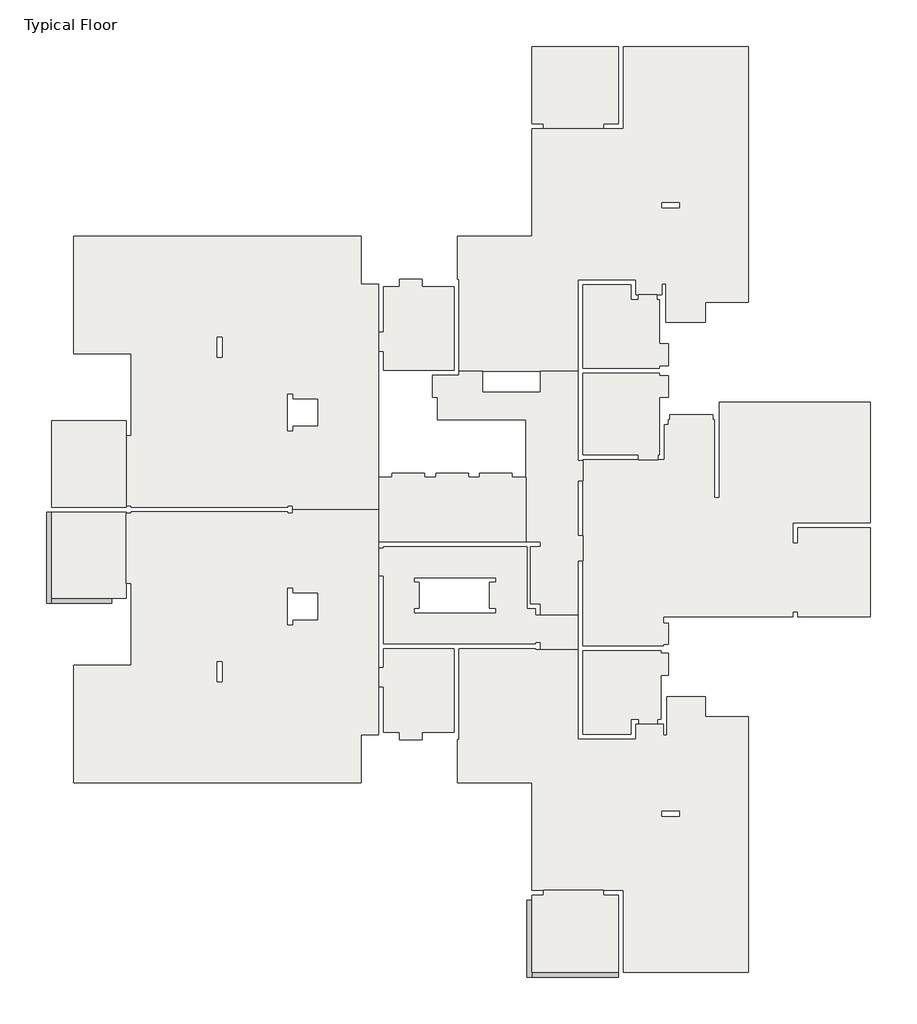
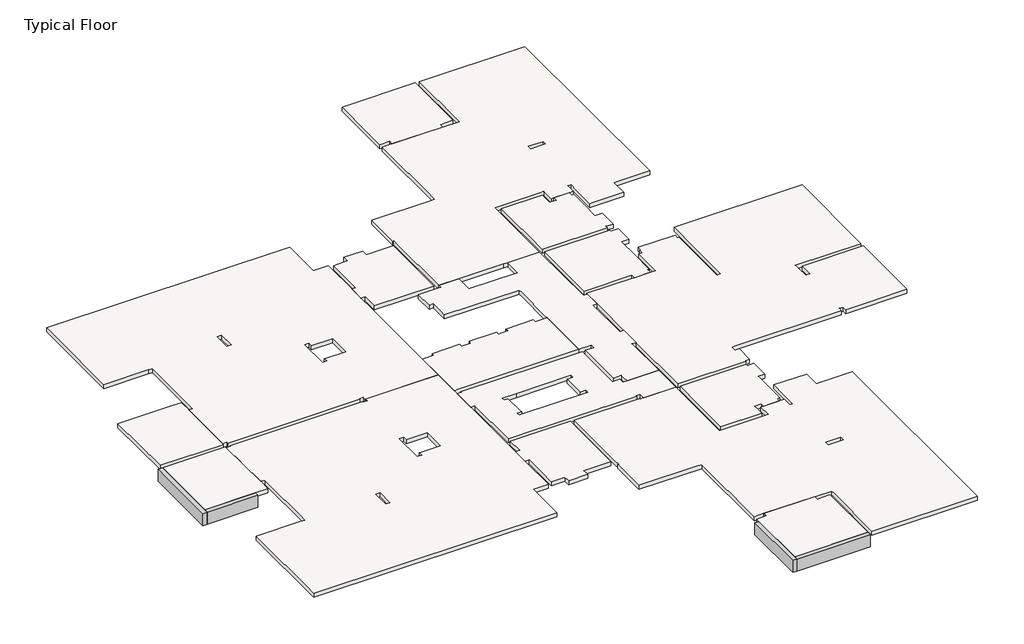
# One storey: 17 slabs, 4 beams.
"""IFC4 building model written with IfcOpenShell, lengths in millimetres."""

from ifc_helpers import new_model, si_unit, frame, origin, place, context, project, spatial, polyline, outline, extrude, faceted_brep, element, save

model = new_model("IFC4")

# Units and contexts
model_context = context("Model", 3, world=origin())
ifc_project = project(units=[si_unit("LENGTHUNIT", "METRE", prefix="MILLI")], contexts=[model_context])

# Site, building, storey
site = spatial("IfcSite", under=ifc_project)
building = spatial("IfcBuilding", under=site)
storey = spatial("IfcBuildingStorey", under=building, Name="Typical Floor", Elevation=3000.0)

# Beams
placement = place(None, origin())
element("IfcBeam", 1, ObjectType="Concrete Rectengular Beam : 20/60", at=placement, inside=storey, context=model_context, shape_type="Brep", body=[
    faceted_brep([(-15942.9172386, -82.3626254, 3000.0), (-15742.9172386, -82.3626254, 3000.0), (-15742.9172386, 117.6373746, 3000.0), (-15742.9172386, 3570.6507339, 3000.0), (-15942.9172386, 3570.6507339, 3000.0), (-15742.9172386, -82.3626254, 2400.0), (-15742.9172386, 117.6373746, 2400.0), (-15742.9172386, 3570.6507339, 2400.0), (-15742.9172386, 3570.6507339, 2800.0), (-15942.9172386, -82.3626254, 2400.0), (-15942.9172386, 3570.6507339, 2400.0)], [[[0, 1, 2, 3, 4]], [[1, 5, 6, 7, 8, 3, 2]], [[5, 9, 10, 7, 6]], [[9, 0, 4, 10]], [[1, 0, 9, 5]], [[4, 3, 8, 7, 10]]]),
])
element("IfcBeam", 2, ObjectType="Concrete Rectengular Beam : 20/60", at=placement, inside=storey, context=model_context, shape_type="Brep", body=[
    faceted_brep([(-15742.9172386, 117.6373746, 3000.0), (-15742.9172386, -82.3626254, 3000.0), (-13340.0412254, -82.3626254, 3000.0), (-13340.0412254, 117.6373746, 3000.0), (-15742.9172386, 117.6373746, 2400.0), (-15742.9172386, 117.6373746, 2800.0), (-13340.0412254, 117.6373746, 2400.0), (-15742.9172386, -82.3626254, 2400.0), (-13340.0412254, -82.3626254, 2400.0)], [[[0, 1, 2, 3]], [[4, 5, 0, 3, 6]], [[7, 4, 6, 8]], [[8, 2, 1, 7]], [[1, 0, 5, 4, 7]], [[3, 2, 8, 6]]]),
])
element("IfcBeam", 3, ObjectType="Concrete Rectengular Beam : 20/60", at=placement, inside=storey, context=model_context, shape_type="Brep", body=[
    faceted_brep([(3325.3580541, -15077.7243787, 3000.0), (3525.3580541, -15077.7243787, 3000.0), (3525.3580541, -14877.7243787, 3000.0), (3525.3580541, -11977.8894943, 3000.0), (3325.3580541, -11977.8894943, 3000.0), (3525.3580541, -15077.7243787, 2400.0), (3525.3580541, -14877.7243787, 2400.0), (3525.3580541, -11977.8894943, 2400.0), (3325.3580541, -15077.7243787, 2400.0), (3325.3580541, -11977.8894943, 2400.0)], [[[0, 1, 2, 3, 4]], [[1, 5, 6, 7, 3, 2]], [[5, 8, 9, 7, 6]], [[8, 0, 4, 9]], [[1, 0, 8, 5]], [[4, 3, 7, 9]]]),
])
element("IfcBeam", 4, ObjectType="Concrete Rectengular Beam : 20/60", at=placement, inside=storey, context=model_context, shape_type="Brep", body=[
    faceted_brep([(6985.0248209, -15077.7243787, 3000.0), (6985.0248209, -14877.7243787, 3000.0), (3525.3580541, -14877.7243787, 3000.0), (3525.3580541, -15077.7243787, 3000.0), (6985.0248209, -14877.7243787, 2800.0), (6985.0248209, -14877.7243787, 2400.0), (3525.3580541, -14877.7243787, 2400.0), (3525.3580541, -14877.7243787, 2800.0), (6985.0248209, -15077.7243787, 2400.0), (3525.3580541, -15077.7243787, 2400.0)], [[[0, 1, 2, 3]], [[1, 4, 5, 6, 7, 2]], [[5, 8, 9, 6]], [[8, 0, 3, 9]], [[1, 0, 8, 5, 4]], [[3, 2, 7, 6, 9]]]),
])

# Slabs
element("IfcSlab", 5, ObjectType="20", at=placement, inside=storey, context=model_context, shape_type="Brep", body=[
    faceted_brep([(-12744.8761098, 117.6373746, 2800.0), (-15742.9172386, 117.6373746, 2800.0), (-15742.9172386, 3570.6507339, 2800.0), (-12745.0412254, 3570.6507339, 2800.0), (-12745.0412254, 3522.8272575, 2800.0), (-12744.8761098, 3522.8272575, 2800.0), (-12744.8761098, 723.063673, 2800.0), (-15742.9172386, 117.6373746, 3000.0), (-13340.0412254, 117.6373746, 3000.0), (-12744.8761098, 117.6373746, 3000.0), (-12744.8761098, 723.063673, 3000.0), (-12744.8761098, 3522.8272575, 3000.0), (-12745.0412254, 3522.8272575, 3000.0), (-12745.0412254, 3570.6507339, 3000.0), (-15742.9172386, 3570.6507339, 3000.0)], [[[0, 1, 2, 3, 4, 5, 6]], [[7, 8, 9, 10, 11, 12, 13, 14]], [[9, 0, 6, 5, 11, 10]], [[1, 0, 9, 8, 7]], [[2, 1, 7, 14]], [[2, 14, 13, 3]], [[12, 4, 3, 13]], [[4, 12, 11, 5]]]),
])
element("IfcSlab", 6, ObjectType="20", at=placement, inside=storey, context=model_context, shape_type="Brep", body=[
    faceted_brep([(-15742.9172386, 3770.6507339, 2800.0), (-15742.9172386, 7228.4299293, 2800.0), (-12744.8761098, 7228.4299293, 2800.0), (-12744.8761098, 6623.0036309, 2800.0), (-12742.9172386, 6623.0036309, 2800.0), (-12742.9172386, 3823.2400464, 2800.0), (-12742.9172386, 3818.3090948, 2800.0), (-12745.0412254, 3818.3090948, 2800.0), (-12745.0412254, 3770.6507339, 2800.0), (-15742.9172386, 7228.4299293, 3000.0), (-15742.9172386, 3770.6507339, 3000.0), (-12745.0412254, 3770.6507339, 3000.0), (-12745.0412254, 3818.3090948, 3000.0), (-12742.9172386, 3818.3090948, 3000.0), (-12742.9172386, 3823.2400464, 3000.0), (-12742.9172386, 6623.0036309, 3000.0), (-12744.8761098, 6623.0036309, 3000.0), (-12744.8761098, 7228.4299293, 3000.0), (-13340.0412254, 7228.4299293, 3000.0)], [[[0, 1, 2, 3, 4, 5, 6, 7, 8]], [[9, 10, 11, 12, 13, 14, 15, 16, 17, 18]], [[4, 15, 14, 13, 6, 5]], [[10, 0, 8, 11]], [[1, 0, 10, 9]], [[1, 9, 18, 17, 2]], [[16, 3, 2, 17]], [[3, 16, 15, 4]], [[7, 12, 11, 8]], [[12, 7, 6, 13]]]),
])
element("IfcSlab", 7, ObjectType="20", at=placement, inside=storey, context=model_context, shape_type="Brep", body=[
    faceted_brep([(-12744.8761098, 3522.8272575, 2800.0), (-12545.0412254, 3522.8272575, 2800.0), (-12545.0412254, 3573.033652, 2800.0), (-6284.9504118, 3573.033652, 2800.0), (-6284.9504118, 3522.8272575, 2800.0), (-6084.9504118, 3522.8272575, 2800.0), (-6084.9504118, 3672.9510942, 2800.0), (-2634.3199705, 3672.9510942, 2800.0), (-2634.3199705, 2374.2607609, 2800.0), (-2634.3199705, 2124.0543665, 2800.0), (-2634.3199705, 1012.4872695, 2800.0), (-2634.3199705, -2660.6799476, 2800.0), (-2634.3199705, -3430.3624753, 2800.0), (-2634.3199705, -5346.2285816, 2800.0), (-3134.897875, -5346.2285816, 2800.0), (-3334.897875, -5346.2285816, 2800.0), (-3334.897875, -7276.5573117, 2800.0), (-14851.7058906, -7276.5573117, 2800.0), (-14851.7058906, -2576.5573117, 2800.0), (-12744.8761098, -2576.5573117, 2800.0), (-12744.8761098, -2576.936327, 2800.0), (-12544.8761098, -2576.936327, 2800.0), (-12544.8761098, 723.063673, 2800.0), (-12744.8761098, 723.063673, 2800.0), (-8908.7851697, -2433.7684532, 2800.0), (-9108.7851697, -2433.7684532, 2800.0), (-9108.7851697, -3233.7684532, 2800.0), (-8908.7851697, -3233.7684532, 2800.0), (-6084.7852962, 522.8985574, 2800.0), (-6284.7852962, 522.8985574, 2800.0), (-6284.7852962, -947.1014426, 2800.0), (-6084.7852962, -947.1014426, 2800.0), (-6084.7852962, -744.8138413, 2800.0), (-5083.9597183, -744.8138413, 2800.0), (-5083.9597183, 322.7334418, 2800.0), (-6084.7852962, 322.7334418, 2800.0), (-12545.0412254, 3522.8272575, 3000.0), (-12744.8761098, 3522.8272575, 3000.0), (-12744.8761098, 723.063673, 3000.0), (-12544.8761098, 723.063673, 3000.0), (-12544.8761098, -2576.936327, 3000.0), (-12744.8761098, -2576.936327, 3000.0), (-12744.8761098, -2576.5573117, 3000.0), (-14851.7058906, -2576.5573117, 3000.0), (-14851.7058906, -7276.5573117, 3000.0), (-3334.897875, -7276.5573117, 3000.0), (-3334.897875, -5346.2285816, 3000.0), (-3134.897875, -5346.2285816, 3000.0), (-2634.3199705, -5346.2285816, 3000.0), (-2634.3199705, -3430.3624753, 3000.0), (-2634.3199705, -2660.6799476, 3000.0), (-2634.3199705, 1012.4872695, 3000.0), (-2634.3199705, 2124.0543665, 3000.0), (-2634.3199705, 2374.2607609, 3000.0), (-2634.3199705, 3672.9510942, 3000.0), (-6084.9504118, 3672.9510942, 3000.0), (-6084.9504118, 3522.8272575, 3000.0), (-6284.9504118, 3522.8272575, 3000.0), (-6284.9504118, 3573.033652, 3000.0), (-12545.0412254, 3573.033652, 3000.0), (-9108.7851697, -2433.7684532, 3000.0), (-8908.7851697, -2433.7684532, 3000.0), (-8908.7851697, -3233.7684532, 3000.0), (-9108.7851697, -3233.7684532, 3000.0), (-6284.7852962, 522.8985574, 3000.0), (-6084.7852962, 522.8985574, 3000.0), (-6084.7852962, 322.7334418, 3000.0), (-5083.9597183, 322.7334418, 3000.0), (-5083.9597183, -744.8138413, 3000.0), (-6084.7852962, -744.8138413, 3000.0), (-6084.7852962, -947.1014426, 3000.0), (-6284.7852962, -947.1014426, 3000.0)], [[[0, 1, 2, 3, 4, 5, 6, 7, 8, 9, 10, 11, 12, 13, 14, 15, 16, 17, 18, 19, 20, 21, 22, 23], [24, 25, 26, 27], [28, 29, 30, 31, 32, 33, 34, 35]], [[36, 37, 38, 39, 40, 41, 42, 43, 44, 45, 46, 47, 48, 49, 50, 51, 52, 53, 54, 55, 56, 57, 58, 59], [60, 61, 62, 63], [64, 65, 66, 67, 68, 69, 70, 71]], [[1, 0, 37, 36]], [[2, 1, 36, 59]], [[3, 2, 59, 58]], [[4, 3, 58, 57]], [[5, 4, 57, 56]], [[6, 5, 56, 55]], [[7, 6, 55, 54]], [[13, 12, 11, 10, 9, 8, 7, 54, 53, 52, 51, 50, 49, 48]], [[13, 48, 47, 46, 15, 14]], [[15, 46, 45, 16]], [[43, 18, 17, 44]], [[18, 43, 42, 19]], [[38, 23, 22, 39]], [[0, 23, 38, 37]], [[25, 24, 61, 60]], [[26, 25, 60, 63]], [[27, 26, 63, 62]], [[24, 27, 62, 61]], [[29, 28, 65, 64]], [[30, 29, 64, 71]], [[31, 30, 71, 70]], [[32, 31, 70, 69]], [[33, 32, 69, 68]], [[34, 33, 68, 67]], [[35, 34, 67, 66]], [[28, 35, 66, 65]], [[21, 40, 39, 22]], [[41, 20, 19, 42]], [[40, 21, 20, 41]], [[17, 16, 45, 44]]]),
])
element("IfcSlab", 8, ObjectType="20", at=placement, inside=storey, context=model_context, shape_type="Brep", body=[
    faceted_brep([(-6284.9504118, 3773.033652, 2800.0), (-12545.0412254, 3773.033652, 2800.0), (-12545.0412254, 3818.3090948, 2800.0), (-12545.0412254, 3823.2400464, 2800.0), (-12742.9172386, 3823.2400464, 2800.0), (-12742.9172386, 6623.0036309, 2800.0), (-12544.8761098, 6623.0036309, 2800.0), (-12544.8761098, 9923.0036309, 2800.0), (-12744.8761098, 9923.0036309, 2800.0), (-12744.8761098, 9922.6246156, 2800.0), (-14851.7058906, 9922.6246156, 2800.0), (-14851.7058906, 14622.6246156, 2800.0), (-3334.897875, 14622.6246156, 2800.0), (-3334.897875, 12692.2958855, 2800.0), (-3134.897875, 12692.2958855, 2800.0), (-2634.3199705, 12692.2958855, 2800.0), (-2634.3199705, 10776.4297792, 2800.0), (-2634.3199705, 10006.7472515, 2800.0), (-2634.3199705, 4974.0243454, 2800.0), (-2634.3199705, 3672.9510942, 2800.0), (-6084.9504118, 3672.9510942, 2800.0), (-6084.9504118, 3823.2400464, 2800.0), (-6284.9504118, 3823.2400464, 2800.0), (-9108.7851697, 9779.8357571, 2800.0), (-8908.7851697, 9779.8357571, 2800.0), (-8908.7851697, 10579.8357571, 2800.0), (-9108.7851697, 10579.8357571, 2800.0), (-6284.7852962, 6823.1687465, 2800.0), (-6084.7852962, 6823.1687465, 2800.0), (-6084.7852962, 7023.3338621, 2800.0), (-5083.9597183, 7023.3338621, 2800.0), (-5083.9597183, 8090.8811452, 2800.0), (-6084.7852962, 8090.8811452, 2800.0), (-6084.7852962, 8293.1687465, 2800.0), (-6284.7852962, 8293.1687465, 2800.0), (-12545.0412254, 3773.033652, 3000.0), (-6284.9504118, 3773.033652, 3000.0), (-6284.9504118, 3823.2400464, 3000.0), (-6084.9504118, 3823.2400464, 3000.0), (-6084.9504118, 3672.9510942, 3000.0), (-2634.3199705, 3672.9510942, 3000.0), (-2634.3199705, 4974.0243454, 3000.0), (-2634.3199705, 5124.0243454, 3000.0), (-2634.3199705, 7974.2832767, 3000.0), (-2634.3199705, 8174.2832767, 3000.0), (-2634.3199705, 9053.5800344, 3000.0), (-2634.3199705, 9253.5800344, 3000.0), (-2634.3199705, 10006.7472515, 3000.0), (-2634.3199705, 10776.4297792, 3000.0), (-2634.3199705, 12692.2958855, 3000.0), (-3134.897875, 12692.2958855, 3000.0), (-3334.897875, 12692.2958855, 3000.0), (-3334.897875, 14622.6246156, 3000.0), (-14851.7058906, 14622.6246156, 3000.0), (-14851.7058906, 9922.6246156, 3000.0), (-12744.8761098, 9922.6246156, 3000.0), (-12744.8761098, 9923.0036309, 3000.0), (-12544.8761098, 9923.0036309, 3000.0), (-12544.8761098, 6623.0036309, 3000.0), (-12742.9172386, 6623.0036309, 3000.0), (-12742.9172386, 3823.2400464, 3000.0), (-12545.0412254, 3823.2400464, 3000.0), (-12545.0412254, 3818.3090948, 3000.0), (-8908.7851697, 9779.8357571, 3000.0), (-9108.7851697, 9779.8357571, 3000.0), (-9108.7851697, 10579.8357571, 3000.0), (-8908.7851697, 10579.8357571, 3000.0), (-6084.7852962, 6823.1687465, 3000.0), (-6284.7852962, 6823.1687465, 3000.0), (-6284.7852962, 8293.1687465, 3000.0), (-6084.7852962, 8293.1687465, 3000.0), (-6084.7852962, 8090.8811452, 3000.0), (-5083.9597183, 8090.8811452, 3000.0), (-5083.9597183, 7023.3338621, 3000.0), (-6084.7852962, 7023.3338621, 3000.0)], [[[0, 1, 2, 3, 4, 5, 6, 7, 8, 9, 10, 11, 12, 13, 14, 15, 16, 17, 18, 19, 20, 21, 22], [23, 24, 25, 26], [27, 28, 29, 30, 31, 32, 33, 34]], [[35, 36, 37, 38, 39, 40, 41, 42, 43, 44, 45, 46, 47, 48, 49, 50, 51, 52, 53, 54, 55, 56, 57, 58, 59, 60, 61, 62], [63, 64, 65, 66], [67, 68, 69, 70, 71, 72, 73, 74]], [[3, 61, 60, 4]], [[1, 35, 62, 61, 3, 2]], [[1, 0, 36, 35]], [[0, 22, 37, 36]], [[22, 21, 38, 37]], [[21, 20, 39, 38]], [[20, 19, 40, 39]], [[19, 18, 17, 16, 15, 49, 48, 47, 46, 45, 44, 43, 42, 41, 40]], [[13, 51, 50, 49, 15, 14]], [[51, 13, 12, 52]], [[10, 54, 53, 11]], [[54, 10, 9, 55]], [[58, 6, 5, 59]], [[24, 23, 64, 63]], [[23, 26, 65, 64]], [[26, 25, 66, 65]], [[25, 24, 63, 66]], [[28, 27, 68, 67]], [[27, 34, 69, 68]], [[34, 33, 70, 69]], [[33, 32, 71, 70]], [[32, 31, 72, 71]], [[31, 30, 73, 72]], [[30, 29, 74, 73]], [[29, 28, 67, 74]], [[8, 56, 55, 9]], [[6, 58, 57, 7]], [[7, 57, 56, 8]], [[5, 4, 60, 59]], [[12, 11, 53, 52]]]),
])
element("IfcSlab", 9, ObjectType="20", at=placement, inside=storey, context=model_context, shape_type="SweptSolid", body=[
    extrude(outline(polyline([(-2434.3199705, -2660.6799476), (-2434.3199705, -1909.5654174), (385.0023051, -1909.5654174), (385.0023051, -5246.2285816), (-885.2581272, -5246.2285816), (-885.2581272, -5546.2285816), (-1781.9370524, -5546.2285816), (-1781.9370524, -5246.2285816), (-2434.3199705, -5246.2285816), (-2434.3199705, -3430.3624753), (-2634.3199705, -3430.3624753), (-2634.3199705, -2660.6799476), (-2434.3199705, -2660.6799476)])), frame((0.0, 0.0, 2800.0), z_axis=(0.0, 0.0, 1.0), x_axis=(1.0, 0.0, 0.0)), (0.0, 0.0, 1.0), 200.0),
])
element("IfcSlab", 10, ObjectType="20", at=placement, inside=storey, context=model_context, shape_type="Brep", body=[
    faceted_brep([(3654.3658596, -1909.5654174, 2800.0), (3654.3658596, -1955.5013225, 2800.0), (3854.3658596, -1955.5013225, 2800.0), (5355.6042265, -1955.5013225, 2800.0), (5355.6042265, -5329.7132709, 2800.0), (5355.6042265, -5529.7132709, 2800.0), (7481.1671205, -5529.7132709, 2800.0), (7681.1671205, -5529.7132709, 2800.0), (7681.1671205, -4929.2179242, 2800.0), (7809.9023103, -4929.2179242, 2800.0), (8554.8987326, -4929.2179242, 2800.0), (8779.8987326, -4929.2179242, 2800.0), (8779.8987326, -5377.2065162, 2800.0), (8929.8987326, -5377.2065162, 2800.0), (8929.8987326, -4829.2179242, 2800.0), (8929.8987326, -3825.7617548, 2800.0), (10478.8780181, -3825.7617548, 2800.0), (10478.8780181, -4426.5873327, 2800.0), (10478.8780181, -4626.5873327, 2800.0), (12185.0248209, -4626.5873327, 2800.0), (12185.0248209, -14877.7243787, 2800.0), (7185.0248209, -14877.7243787, 2800.0), (7185.0248209, -11777.7243787, 2800.0), (7185.0248209, -11577.7243787, 2800.0), (6385.0248209, -11577.7243787, 2800.0), (3983.0434339, -11577.7243787, 2800.0), (3525.3580541, -11577.7243787, 2800.0), (3525.3580541, -7276.5573117, 2800.0), (539.5617467, -7276.5573117, 2800.0), (539.5617467, -5546.2285816, 2800.0), (585.0023051, -5546.2285816, 2800.0), (585.0023051, -5246.2285816, 2800.0), (585.0023051, -1909.5654174, 2800.0), (9430.3940793, -8427.3416107, 2800.0), (8730.3940793, -8427.3416107, 2800.0), (8730.3940793, -8627.3416107, 2800.0), (9430.3940793, -8627.3416107, 2800.0), (3654.3658596, -1955.5013225, 3000.0), (3654.3658596, -1909.5654174, 3000.0), (585.0023051, -1909.5654174, 3000.0), (585.0023051, -5246.2285816, 3000.0), (585.0023051, -5546.2285816, 3000.0), (539.5617467, -5546.2285816, 3000.0), (539.5617467, -7276.5573117, 3000.0), (3325.3580541, -7276.5573117, 3000.0), (3525.3580541, -7276.5573117, 3000.0), (3525.3580541, -11577.7243787, 3000.0), (3983.0434339, -11577.7243787, 3000.0), (6385.0248209, -11577.7243787, 3000.0), (7185.0248209, -11577.7243787, 3000.0), (7185.0248209, -11777.7243787, 3000.0), (7185.0248209, -14877.7243787, 3000.0), (12185.0248209, -14877.7243787, 3000.0), (12185.0248209, -4626.5873327, 3000.0), (10478.8780181, -4626.5873327, 3000.0), (10478.8780181, -4426.5873327, 3000.0), (10478.8780181, -3825.7617548, 3000.0), (8929.8987326, -3825.7617548, 3000.0), (8929.8987326, -4829.2179242, 3000.0), (8929.8987326, -5377.2065162, 3000.0), (8779.8987326, -5377.2065162, 3000.0), (8779.8987326, -4929.2179242, 3000.0), (8554.8987326, -4929.2179242, 3000.0), (7809.9023103, -4929.2179242, 3000.0), (7681.1671205, -4929.2179242, 3000.0), (7681.1671205, -5529.7132709, 3000.0), (7481.1671205, -5529.7132709, 3000.0), (5355.6042265, -5529.7132709, 3000.0), (5355.6042265, -5329.7132709, 3000.0), (5355.6042265, -1955.5013225, 3000.0), (3854.3658596, -1955.5013225, 3000.0), (8730.3940793, -8427.3416107, 3000.0), (9430.3940793, -8427.3416107, 3000.0), (9430.3940793, -8627.3416107, 3000.0), (8730.3940793, -8627.3416107, 3000.0)], [[[0, 1, 2, 3, 4, 5, 6, 7, 8, 9, 10, 11, 12, 13, 14, 15, 16, 17, 18, 19, 20, 21, 22, 23, 24, 25, 26, 27, 28, 29, 30, 31, 32], [33, 34, 35, 36]], [[37, 38, 39, 40, 41, 42, 43, 44, 45, 46, 47, 48, 49, 50, 51, 52, 53, 54, 55, 56, 57, 58, 59, 60, 61, 62, 63, 64, 65, 66, 67, 68, 69, 70], [71, 72, 73, 74]], [[1, 0, 38, 37]], [[2, 1, 37, 70]], [[3, 2, 70, 69]], [[3, 69, 68, 67, 5, 4]], [[5, 67, 66, 65, 7, 6]], [[8, 7, 65, 64]], [[8, 64, 63, 62, 61, 11, 10, 9]], [[12, 11, 61, 60]], [[13, 12, 60, 59]], [[13, 59, 58, 57, 15, 14]], [[16, 15, 57, 56]], [[16, 56, 55, 54, 18, 17]], [[19, 18, 54, 53]], [[20, 19, 53, 52]], [[21, 20, 52, 51]], [[21, 51, 50, 49, 23, 22]], [[24, 23, 49, 48]], [[25, 24, 48, 47]], [[26, 25, 47, 46]], [[26, 46, 45, 27]], [[42, 29, 28, 43]], [[30, 29, 42, 41]], [[30, 41, 40, 39, 32, 31]], [[0, 32, 39, 38]], [[34, 33, 72, 71]], [[35, 34, 71, 74]], [[36, 35, 74, 73]], [[33, 36, 73, 72]], [[27, 45, 44, 43, 28]]]),
])
element("IfcSlab", 11, ObjectType="20", at=placement, inside=storey, context=model_context, shape_type="Brep", body=[
    faceted_brep([(3983.0434339, -11777.7243787, 2800.0), (3983.0434339, -11577.7243787, 2800.0), (6385.0248209, -11577.7243787, 2800.0), (6385.0248209, -11777.7243787, 2800.0), (6985.0248209, -11777.7243787, 2800.0), (6985.0248209, -14877.7243787, 2800.0), (3525.3580541, -14877.7243787, 2800.0), (3525.3580541, -11777.7243787, 2800.0), (3983.0434339, -11577.7243787, 3000.0), (3983.0434339, -11777.7243787, 3000.0), (3525.3580541, -11777.7243787, 3000.0), (3525.3580541, -11977.8894943, 3000.0), (3525.3580541, -14877.7243787, 3000.0), (6985.0248209, -14877.7243787, 3000.0), (6985.0248209, -11777.7243787, 3000.0), (6385.0248209, -11777.7243787, 3000.0), (6385.0248209, -11577.7243787, 3000.0)], [[[0, 1, 2, 3, 4, 5, 6, 7]], [[8, 9, 10, 11, 12, 13, 14, 15, 16]], [[1, 0, 9, 8]], [[2, 1, 8, 16]], [[3, 2, 16, 15]], [[4, 3, 15, 14]], [[5, 4, 14, 13]], [[6, 5, 13, 12]], [[7, 6, 12, 11, 10]], [[0, 7, 10, 9]]]),
])
element("IfcSlab", 12, ObjectType="20", at=placement, inside=storey, context=model_context, shape_type="Brep", body=[
    faceted_brep([(8680.0225693, -4729.2179242, 2800.0), (8554.8987326, -4729.2179242, 2800.0), (8554.8987326, -4929.2179242, 2800.0), (7809.9023103, -4929.2179242, 2800.0), (7809.9023103, -4729.2179242, 2800.0), (7481.1671205, -4729.2179242, 2800.0), (7481.1671205, -4929.2179242, 2800.0), (7481.1671205, -5329.7132709, 2800.0), (5555.6042265, -5329.7132709, 2800.0), (5555.6042265, -1979.0002718, 2800.0), (8679.7748959, -1979.0002718, 2800.0), (8679.7748959, -2077.0301427, 2800.0), (8979.7748959, -2077.0301427, 2800.0), (8979.7748959, -2977.6080472, 2800.0), (8679.7748959, -2977.6080472, 2800.0), (8679.7748959, -3625.7617548, 2800.0), (8680.0225693, -3625.7617548, 2800.0), (8680.0225693, -3825.7617548, 2800.0), (8554.8987326, -4729.2179242, 3000.0), (8680.0225693, -4729.2179242, 3000.0), (8680.0225693, -3825.7617548, 3000.0), (8680.0225693, -3625.7617548, 3000.0), (8679.7748959, -3625.7617548, 3000.0), (8679.7748959, -2977.6080472, 3000.0), (8979.7748959, -2977.6080472, 3000.0), (8979.7748959, -2077.0301427, 3000.0), (8679.7748959, -2077.0301427, 3000.0), (8679.7748959, -1979.0002718, 3000.0), (5555.6042265, -1979.0002718, 3000.0), (5555.6042265, -5329.7132709, 3000.0), (7481.1671205, -5329.7132709, 3000.0), (7481.1671205, -4929.2179242, 3000.0), (7481.1671205, -4729.2179242, 3000.0), (7809.9023103, -4729.2179242, 3000.0), (7809.9023103, -4929.2179242, 3000.0), (8554.8987326, -4929.2179242, 3000.0)], [[[0, 1, 2, 3, 4, 5, 6, 7, 8, 9, 10, 11, 12, 13, 14, 15, 16, 17]], [[18, 19, 20, 21, 22, 23, 24, 25, 26, 27, 28, 29, 30, 31, 32, 33, 34, 35]], [[19, 0, 17, 16, 21, 20]], [[1, 0, 19, 18]], [[2, 1, 18, 35]], [[3, 2, 35, 34]], [[4, 3, 34, 33]], [[5, 4, 33, 32]], [[5, 32, 31, 30, 7, 6]], [[8, 7, 30, 29]], [[9, 8, 29, 28]], [[10, 9, 28, 27]], [[11, 10, 27, 26]], [[12, 11, 26, 25]], [[13, 12, 25, 24]], [[13, 24, 23, 14]], [[14, 23, 22, 15]], [[15, 22, 21, 16]]]),
])
element("IfcSlab", 13, ObjectType="20", at=placement, inside=storey, context=model_context, shape_type="SweptSolid", body=[
    extrude(outline(polyline([(-885.2581272, 12592.2958855), (385.0023051, 12592.2958855), (385.0023051, 9253.5800344), (-2434.3199705, 9253.5800344), (-2434.3199705, 10006.7472515), (-2634.3199705, 10006.7472515), (-2634.3199705, 10776.4297792), (-2434.3199705, 10776.4297792), (-2434.3199705, 12592.2958855), (-1781.9370524, 12592.2958855), (-1781.9370524, 12892.2958855), (-885.2581272, 12892.2958855), (-885.2581272, 12592.2958855)])), frame((0.0, 0.0, 2800.0), z_axis=(0.0, 0.0, 1.0), x_axis=(1.0, 0.0, 0.0)), (0.0, 0.0, 1.0), 200.0),
])
element("IfcSlab", 14, ObjectType="20", at=placement, inside=storey, context=model_context, shape_type="Brep", body=[
    faceted_brep([(3854.3658596, 9203.7038711, 2800.0), (3654.3658596, 9203.7038711, 2800.0), (1535.7866041, 9203.7038711, 2800.0), (585.0023051, 9203.7038711, 2800.0), (585.0023051, 12592.2958855, 2800.0), (585.0023051, 12892.2958855, 2800.0), (539.5617467, 12892.2958855, 2800.0), (539.5617467, 14622.6246156, 2800.0), (3525.3580541, 14622.6246156, 2800.0), (3525.3580541, 18923.7916826, 2800.0), (3983.0434339, 18923.7916826, 2800.0), (6385.0248209, 18923.7916826, 2800.0), (7185.0248209, 18923.7916826, 2800.0), (7185.0248209, 19123.7916826, 2800.0), (7185.0248209, 22223.7916826, 2800.0), (12185.0248209, 22223.7916826, 2800.0), (12185.0248209, 11972.6546366, 2800.0), (10478.8780181, 11972.6546366, 2800.0), (10478.8780181, 11772.6546366, 2800.0), (10478.8780181, 11171.8290587, 2800.0), (8979.733617, 11171.8290587, 2800.0), (8879.6510592, 11171.8290587, 2800.0), (8879.6510592, 12075.1201125, 2800.0), (8879.6510592, 12275.1201125, 2800.0), (8879.6510592, 12723.2738201, 2800.0), (8729.6510592, 12723.2738201, 2800.0), (8729.6510592, 12275.1201125, 2800.0), (8530.0225693, 12275.1201125, 2800.0), (8530.0225693, 12270.1201125, 2800.0), (7795.7123021, 12270.1201125, 2800.0), (7795.7123021, 12275.2852281, 2800.0), (7681.1671205, 12275.2852281, 2800.0), (7681.1671205, 12875.7805748, 2800.0), (7481.1671205, 12875.7805748, 2800.0), (5355.6042265, 12875.7805748, 2800.0), (5355.6042265, 12675.7805748, 2800.0), (5355.6042265, 9203.7038711, 2800.0), (8730.3940793, 15773.4089146, 2800.0), (9430.3940793, 15773.4089146, 2800.0), (9430.3940793, 15973.4089146, 2800.0), (8730.3940793, 15973.4089146, 2800.0), (3654.3658596, 9203.7038711, 3000.0), (3854.3658596, 9203.7038711, 3000.0), (5355.6042265, 9203.7038711, 3000.0), (5355.6042265, 12675.7805748, 3000.0), (5355.6042265, 12875.7805748, 3000.0), (7481.1671205, 12875.7805748, 3000.0), (7681.1671205, 12875.7805748, 3000.0), (7681.1671205, 12275.2852281, 3000.0), (7795.7123021, 12275.2852281, 3000.0), (7795.7123021, 12270.1201125, 3000.0), (8530.0225693, 12270.1201125, 3000.0), (8530.0225693, 12275.1201125, 3000.0), (8729.6510592, 12275.1201125, 3000.0), (8729.6510592, 12723.2738201, 3000.0), (8879.6510592, 12723.2738201, 3000.0), (8879.6510592, 12275.1201125, 3000.0), (8879.6510592, 12075.1201125, 3000.0), (8879.6510592, 11171.8290587, 3000.0), (8979.733617, 11171.8290587, 3000.0), (10478.8780181, 11171.8290587, 3000.0), (10478.8780181, 11772.6546366, 3000.0), (10478.8780181, 11972.6546366, 3000.0), (12185.0248209, 11972.6546366, 3000.0), (12185.0248209, 22223.7916826, 3000.0), (7185.0248209, 22223.7916826, 3000.0), (7185.0248209, 19123.7916826, 3000.0), (7185.0248209, 18923.7916826, 3000.0), (6385.0248209, 18923.7916826, 3000.0), (3983.0434339, 18923.7916826, 3000.0), (3525.3580541, 18923.7916826, 3000.0), (3525.3580541, 14622.6246156, 3000.0), (3325.3580541, 14622.6246156, 3000.0), (539.5617467, 14622.6246156, 3000.0), (539.5617467, 12892.2958855, 3000.0), (585.0023051, 12892.2958855, 3000.0), (585.0023051, 12592.2958855, 3000.0), (585.0023051, 9203.7038711, 3000.0), (1535.7866041, 9203.7038711, 3000.0), (9430.3940793, 15773.4089146, 3000.0), (8730.3940793, 15773.4089146, 3000.0), (8730.3940793, 15973.4089146, 3000.0), (9430.3940793, 15973.4089146, 3000.0)], [[[0, 1, 2, 3, 4, 5, 6, 7, 8, 9, 10, 11, 12, 13, 14, 15, 16, 17, 18, 19, 20, 21, 22, 23, 24, 25, 26, 27, 28, 29, 30, 31, 32, 33, 34, 35, 36], [37, 38, 39, 40]], [[41, 42, 43, 44, 45, 46, 47, 48, 49, 50, 51, 52, 53, 54, 55, 56, 57, 58, 59, 60, 61, 62, 63, 64, 65, 66, 67, 68, 69, 70, 71, 72, 73, 74, 75, 76, 77, 78], [79, 80, 81, 82]], [[1, 0, 42, 41]], [[0, 36, 43, 42]], [[34, 45, 44, 43, 36, 35]], [[32, 47, 46, 45, 34, 33]], [[47, 32, 31, 48]], [[50, 29, 28, 51]], [[25, 54, 53, 26]], [[25, 24, 55, 54]], [[21, 58, 57, 56, 55, 24, 23, 22]], [[19, 60, 59, 58, 21, 20]], [[17, 62, 61, 60, 19, 18]], [[17, 16, 63, 62]], [[16, 15, 64, 63]], [[15, 14, 65, 64]], [[12, 67, 66, 65, 14, 13]], [[12, 11, 68, 67]], [[11, 10, 69, 68]], [[10, 9, 70, 69]], [[70, 9, 8, 71]], [[6, 74, 73, 7]], [[6, 5, 75, 74]], [[3, 77, 76, 75, 5, 4]], [[3, 2, 1, 41, 78, 77]], [[38, 37, 80, 79]], [[37, 40, 81, 80]], [[40, 39, 82, 81]], [[39, 38, 79, 82]], [[30, 49, 48, 31]], [[49, 30, 29, 50]], [[52, 27, 26, 53]], [[27, 52, 51, 28]], [[71, 8, 7, 73, 72]]]),
])
element("IfcSlab", 15, ObjectType="20", at=placement, inside=storey, context=model_context, shape_type="Brep", body=[
    faceted_brep([(3983.0434339, 18923.7916826, 2800.0), (3983.0434339, 19123.7916826, 2800.0), (3525.3580541, 19123.7916826, 2800.0), (3525.3580541, 22223.7916826, 2800.0), (6985.0248209, 22223.7916826, 2800.0), (6985.0248209, 19123.7916826, 2800.0), (6385.0248209, 19123.7916826, 2800.0), (6385.0248209, 18923.7916826, 2800.0), (3983.0434339, 19123.7916826, 3000.0), (3983.0434339, 18923.7916826, 3000.0), (6385.0248209, 18923.7916826, 3000.0), (6385.0248209, 19123.7916826, 3000.0), (6985.0248209, 19123.7916826, 3000.0), (6985.0248209, 22223.7916826, 3000.0), (3525.3580541, 22223.7916826, 3000.0), (3525.3580541, 19323.9567982, 3000.0), (3525.3580541, 19123.7916826, 3000.0)], [[[0, 1, 2, 3, 4, 5, 6, 7]], [[8, 9, 10, 11, 12, 13, 14, 15, 16]], [[1, 0, 9, 8]], [[0, 7, 10, 9]], [[7, 6, 11, 10]], [[6, 5, 12, 11]], [[5, 4, 13, 12]], [[4, 3, 14, 13]], [[3, 2, 16, 15, 14]], [[2, 1, 8, 16]]]),
])
element("IfcSlab", 16, ObjectType="20", at=placement, inside=storey, context=model_context, shape_type="Brep", body=[
    faceted_brep([(7481.1671205, 12075.2852281, 2800.0), (7795.7123021, 12075.2852281, 2800.0), (7795.7123021, 12270.1201125, 2800.0), (8530.0225693, 12270.1201125, 2800.0), (8530.0225693, 12075.1201125, 2800.0), (8629.733617, 12075.1201125, 2800.0), (8629.733617, 11171.8290587, 2800.0), (8629.733617, 10323.6753511, 2800.0), (8979.733617, 10323.6753511, 2800.0), (8979.733617, 9425.3152491, 2800.0), (8629.733617, 9425.3152491, 2800.0), (8629.733617, 9325.0675757, 2800.0), (5555.6042265, 9325.0675757, 2800.0), (5555.6042265, 12675.7805748, 2800.0), (7481.1671205, 12675.7805748, 2800.0), (7481.1671205, 12275.2852281, 2800.0), (7795.7123021, 12075.2852281, 3000.0), (7481.1671205, 12075.2852281, 3000.0), (7481.1671205, 12275.2852281, 3000.0), (7481.1671205, 12675.7805748, 3000.0), (5555.6042265, 12675.7805748, 3000.0), (5555.6042265, 9325.0675757, 3000.0), (8629.733617, 9325.0675757, 3000.0), (8629.733617, 9425.3152491, 3000.0), (8979.733617, 9425.3152491, 3000.0), (8979.733617, 10323.6753511, 3000.0), (8629.733617, 10323.6753511, 3000.0), (8629.733617, 11171.8290587, 3000.0), (8629.733617, 12075.1201125, 3000.0), (8530.0225693, 12075.1201125, 3000.0), (8530.0225693, 12270.1201125, 3000.0), (7795.7123021, 12270.1201125, 3000.0)], [[[0, 1, 2, 3, 4, 5, 6, 7, 8, 9, 10, 11, 12, 13, 14, 15]], [[16, 17, 18, 19, 20, 21, 22, 23, 24, 25, 26, 27, 28, 29, 30, 31]], [[5, 28, 27, 26, 7, 6]], [[29, 4, 3, 30]], [[1, 16, 31, 2]], [[1, 0, 17, 16]], [[14, 19, 18, 17, 0, 15]], [[14, 13, 20, 19]], [[13, 12, 21, 20]], [[21, 12, 11, 22]], [[5, 4, 29, 28]], [[8, 7, 26, 25]], [[9, 8, 25, 24]], [[9, 24, 23, 10]], [[10, 23, 22, 11]], [[3, 2, 31, 30]]]),
])
element("IfcSlab", 17, ObjectType="20", at=placement, inside=storey, context=model_context, shape_type="SweptSolid", body=[
    extrude(outline(polyline([(8629.733617, 9125.0675757), (8629.733617, 9024.9850179), (8979.733617, 9024.9850179), (8979.733617, 8174.2832767), (8629.733617, 8174.2832767), (8629.733617, 7073.375141), (8629.8987326, 7073.375141), (8629.8987326, 5874.60225), (8565.3948299, 5874.60225), (8565.3948299, 5674.60225), (7795.7123021, 5674.60225), (7795.7123021, 5874.60225), (5555.6042265, 5874.60225), (5555.6042265, 9125.0675757), (8629.733617, 9125.0675757)])), frame((0.0, 0.0, 2800.0), z_axis=(0.0, 0.0, 1.0), x_axis=(1.0, 0.0, 0.0)), (0.0, 0.0, 1.0), 200.0),
])
element("IfcSlab", 18, ObjectType="20", at=placement, inside=storey, context=model_context, shape_type="Brep", body=[
    faceted_brep([(10774.0296242, 7473.7053722, 2800.0), (10774.0296242, 7273.7053722, 2800.0), (10824.7313654, 7273.7053722, 2800.0), (10824.7313654, 4144.7688666, 2800.0), (11024.7313654, 4144.7688666, 2800.0), (11024.7313654, 7974.2832767, 2800.0), (17074.9602757, 7974.2832767, 2800.0), (17074.9602757, 3143.7781731, 2800.0), (13974.6187866, 3143.7781731, 2800.0), (13974.6187866, 2943.7781731, 2800.0), (13974.6187866, 2314.6878099, 2800.0), (14174.6187866, 2314.6878099, 2800.0), (14174.6187866, 2943.7781731, 2800.0), (17074.9602757, 2943.7781731, 2800.0), (17074.9602757, -628.2159728, 2800.0), (14174.6187866, -628.2159728, 2800.0), (14174.6187866, -425.6679392, 2800.0), (13974.6187866, -425.6679392, 2800.0), (13974.6187866, -628.2159728, 2800.0), (8979.8574537, -628.2159728, 2800.0), (8779.8574537, -628.2159728, 2800.0), (8779.8574537, -878.4223673, 2800.0), (8979.8574537, -878.4223673, 2800.0), (8979.8574537, -1726.7411904, 2800.0), (8779.7748959, -1726.7411904, 2800.0), (8779.7748959, -1779.0002718, 2800.0), (5555.6042265, -1779.0002718, 2800.0), (5555.6042265, 1623.6415775, 2800.0), (5555.6042265, 2624.4671554, 2800.0), (5555.6042265, 4823.9005088, 2800.0), (5555.6042265, 5624.5609711, 2800.0), (5555.6042265, 5674.60225, 2800.0), (7795.7123021, 5674.60225, 2800.0), (8565.3948299, 5674.60225, 2800.0), (8829.8987326, 5674.60225, 2800.0), (8829.8987326, 5874.60225, 2800.0), (8829.8987326, 7073.375141, 2800.0), (8979.733617, 7073.375141, 2800.0), (8979.733617, 7273.7053722, 2800.0), (9040.0225693, 7273.7053722, 2800.0), (9040.0225693, 7473.7053722, 2800.0), (10774.0296242, 7273.7053722, 3000.0), (10774.0296242, 7473.7053722, 3000.0), (9040.0225693, 7473.7053722, 3000.0), (9040.0225693, 7273.7053722, 3000.0), (8979.733617, 7273.7053722, 3000.0), (8979.733617, 7073.375141, 3000.0), (8829.8987326, 7073.375141, 3000.0), (8829.8987326, 5874.60225, 3000.0), (8829.8987326, 5674.60225, 3000.0), (8565.3948299, 5674.60225, 3000.0), (7795.7123021, 5674.60225, 3000.0), (5555.6042265, 5674.60225, 3000.0), (5555.6042265, 5624.5609711, 3000.0), (5555.6042265, 4823.9005088, 3000.0), (5555.6042265, 2624.4671554, 3000.0), (5555.6042265, 1623.6415775, 3000.0), (5555.6042265, -1779.0002718, 3000.0), (8779.7748959, -1779.0002718, 3000.0), (8779.7748959, -1726.7411904, 3000.0), (8979.8574537, -1726.7411904, 3000.0), (8979.8574537, -878.4223673, 3000.0), (8779.8574537, -878.4223673, 3000.0), (8779.8574537, -628.2159728, 3000.0), (8979.8574537, -628.2159728, 3000.0), (13974.6187866, -628.2159728, 3000.0), (13974.6187866, -425.6679392, 3000.0), (14174.6187866, -425.6679392, 3000.0), (14174.6187866, -628.2159728, 3000.0), (17074.9602757, -628.2159728, 3000.0), (17074.9602757, 2943.7781731, 3000.0), (14174.6187866, 2943.7781731, 3000.0), (14174.6187866, 2314.6878099, 3000.0), (13974.6187866, 2314.6878099, 3000.0), (13974.6187866, 2943.7781731, 3000.0), (13974.6187866, 3143.7781731, 3000.0), (17074.9602757, 3143.7781731, 3000.0), (17074.9602757, 7974.2832767, 3000.0), (11024.7313654, 7974.2832767, 3000.0), (11024.7313654, 4144.7688666, 3000.0), (10824.7313654, 4144.7688666, 3000.0), (10824.7313654, 7273.7053722, 3000.0)], [[[0, 1, 2, 3, 4, 5, 6, 7, 8, 9, 10, 11, 12, 13, 14, 15, 16, 17, 18, 19, 20, 21, 22, 23, 24, 25, 26, 27, 28, 29, 30, 31, 32, 33, 34, 35, 36, 37, 38, 39, 40]], [[41, 42, 43, 44, 45, 46, 47, 48, 49, 50, 51, 52, 53, 54, 55, 56, 57, 58, 59, 60, 61, 62, 63, 64, 65, 66, 67, 68, 69, 70, 71, 72, 73, 74, 75, 76, 77, 78, 79, 80, 81]], [[1, 0, 42, 41]], [[2, 1, 41, 81]], [[3, 2, 81, 80]], [[4, 3, 80, 79]], [[5, 4, 79, 78]], [[6, 5, 78, 77]], [[7, 6, 77, 76]], [[8, 7, 76, 75]], [[8, 75, 74, 73, 10, 9]], [[11, 10, 73, 72]], [[12, 11, 72, 71]], [[13, 12, 71, 70]], [[14, 13, 70, 69]], [[15, 14, 69, 68]], [[16, 15, 68, 67]], [[17, 16, 67, 66]], [[18, 17, 66, 65]], [[18, 65, 64, 63, 20, 19]], [[21, 20, 63, 62]], [[22, 21, 62, 61]], [[23, 22, 61, 60]], [[24, 23, 60, 59]], [[25, 24, 59, 58]], [[26, 25, 58, 57]], [[31, 30, 29, 28, 27, 26, 57, 56, 55, 54, 53, 52]], [[31, 52, 51, 50, 49, 34, 33, 32]], [[34, 49, 48, 47, 36, 35]], [[37, 36, 47, 46]], [[38, 37, 46, 45]], [[39, 38, 45, 44]], [[40, 39, 44, 43]], [[0, 40, 43, 42]]]),
])
element("IfcSlab", 19, ObjectType="20", at=placement, inside=storey, context=model_context, shape_type="Brep", body=[
    faceted_brep([(-463.4816337, 8174.2832767, 2800.0), (-463.4816337, 9053.5800344, 2800.0), (385.0023051, 9053.5800344, 2800.0), (585.0023051, 9053.5800344, 2800.0), (585.0023051, 9203.7038711, 2800.0), (1535.7866041, 9203.7038711, 2800.0), (1535.7866041, 8374.4483923, 2800.0), (3854.3658596, 8374.4483923, 2800.0), (3854.3658596, 9203.7038711, 2800.0), (5355.6042265, 9203.7038711, 2800.0), (5355.6042265, 5624.5609711, 2800.0), (5555.6042265, 5624.5609711, 2800.0), (5555.6042265, 4823.9005088, 2800.0), (5355.6042265, 4823.9005088, 2800.0), (5355.6042265, 2624.4671554, 2800.0), (5555.6042265, 2624.4671554, 2800.0), (5555.6042265, 1623.6415775, 2800.0), (5355.6042265, 1623.6415775, 2800.0), (5355.6042265, -560.9043547, 2800.0), (3861.0605459, -560.9043547, 2800.0), (3861.0605459, -305.9043547, 2800.0), (3861.0605459, -105.9043547, 2800.0), (3461.0605459, -105.9043547, 2800.0), (3461.0605459, 2174.0956453, 2800.0), (3461.0605459, 2174.2607609, 2800.0), (3861.5146137, 2174.2607609, 2800.0), (3861.5146137, 2374.2607609, 2800.0), (3274.3005639, 2374.2607609, 2800.0), (3274.3005639, 4974.0243454, 2800.0), (3274.3005639, 5124.0243454, 2800.0), (3274.3005639, 7073.375141, 2800.0), (3274.3005639, 7273.375141, 2800.0), (-265.6994361, 7273.375141, 2800.0), (-265.6994361, 7974.2832767, 2800.0), (-265.6994361, 8174.2832767, 2800.0), (-463.4816337, 9053.5800344, 3000.0), (-463.4816337, 8174.2832767, 3000.0), (-265.6994361, 8174.2832767, 3000.0), (-265.6994361, 7974.2832767, 3000.0), (-265.6994361, 7273.375141, 3000.0), (3274.3005639, 7273.375141, 3000.0), (3274.3005639, 7073.375141, 3000.0), (3274.3005639, 5124.0243454, 3000.0), (3274.3005639, 4974.0243454, 3000.0), (3274.3005639, 2374.2607609, 3000.0), (3861.5146137, 2374.2607609, 3000.0), (3861.5146137, 2174.2607609, 3000.0), (3461.0605459, 2174.2607609, 3000.0), (3461.0605459, 2174.0956453, 3000.0), (3461.0605459, -105.9043547, 3000.0), (3861.0605459, -105.9043547, 3000.0), (3861.0605459, -305.9043547, 3000.0), (3861.0605459, -560.9043547, 3000.0), (5355.6042265, -560.9043547, 3000.0), (5355.6042265, 1623.6415775, 3000.0), (5555.6042265, 1623.6415775, 3000.0), (5555.6042265, 2624.4671554, 3000.0), (5355.6042265, 2624.4671554, 3000.0), (5355.6042265, 4823.9005088, 3000.0), (5555.6042265, 4823.9005088, 3000.0), (5555.6042265, 5624.5609711, 3000.0), (5355.6042265, 5624.5609711, 3000.0), (5355.6042265, 9203.7038711, 3000.0), (3854.3658596, 9203.7038711, 3000.0), (3854.3658596, 8374.4483923, 3000.0), (1535.7866041, 8374.4483923, 3000.0), (1535.7866041, 9203.7038711, 3000.0), (585.0023051, 9203.7038711, 3000.0), (585.0023051, 9053.5800344, 3000.0), (385.0023051, 9053.5800344, 3000.0)], [[[0, 1, 2, 3, 4, 5, 6, 7, 8, 9, 10, 11, 12, 13, 14, 15, 16, 17, 18, 19, 20, 21, 22, 23, 24, 25, 26, 27, 28, 29, 30, 31, 32, 33, 34]], [[35, 36, 37, 38, 39, 40, 41, 42, 43, 44, 45, 46, 47, 48, 49, 50, 51, 52, 53, 54, 55, 56, 57, 58, 59, 60, 61, 62, 63, 64, 65, 66, 67, 68, 69]], [[1, 0, 36, 35]], [[1, 35, 69, 68, 3, 2]], [[4, 3, 68, 67]], [[5, 4, 67, 66]], [[6, 5, 66, 65]], [[7, 6, 65, 64]], [[8, 7, 64, 63]], [[9, 8, 63, 62]], [[10, 9, 62, 61]], [[11, 10, 61, 60]], [[12, 11, 60, 59]], [[13, 12, 59, 58]], [[14, 13, 58, 57]], [[15, 14, 57, 56]], [[16, 15, 56, 55]], [[17, 16, 55, 54]], [[18, 17, 54, 53]], [[19, 18, 53, 52]], [[19, 52, 51, 50, 21, 20]], [[22, 21, 50, 49]], [[22, 49, 48, 47, 24, 23]], [[25, 24, 47, 46]], [[26, 25, 46, 45]], [[27, 26, 45, 44]], [[28, 27, 44, 43]], [[28, 43, 42, 41, 40, 31, 30, 29]], [[32, 31, 40, 39]], [[32, 39, 38, 37, 34, 33]], [[0, 34, 37, 36]]]),
])
element("IfcSlab", 20, ObjectType="20", at=placement, inside=storey, context=model_context, shape_type="Brep", body=[
    faceted_brep([(-2083.8659026, 4974.0243454, 2800.0), (-2083.8659026, 5124.0243454, 2800.0), (-785.1755694, 5124.0243454, 2800.0), (-785.1755694, 4974.0243454, 2800.0), (-334.8040593, 4974.0243454, 2800.0), (-334.8040593, 5124.0243454, 2800.0), (966.2691919, 5124.0243454, 2800.0), (966.2691919, 4974.0243454, 2800.0), (1414.2577839, 4974.0243454, 2800.0), (1414.2577839, 5124.0243454, 2800.0), (2715.3310352, 5124.0243454, 2800.0), (2715.3310352, 4974.0243454, 2800.0), (3274.3005639, 4974.0243454, 2800.0), (3274.3005639, 2374.2607609, 2800.0), (-2634.3199705, 2374.2607609, 2800.0), (-2634.3199705, 3672.9510942, 2800.0), (-2634.3199705, 4974.0243454, 2800.0), (-2083.8659026, 5124.0243454, 3000.0), (-2083.8659026, 4974.0243454, 3000.0), (-2634.3199705, 4974.0243454, 3000.0), (-2634.3199705, 3672.9510942, 3000.0), (-2634.3199705, 2374.2607609, 3000.0), (-2434.3199705, 2374.2607609, 3000.0), (3274.3005639, 2374.2607609, 3000.0), (3274.3005639, 4974.0243454, 3000.0), (2715.3310352, 4974.0243454, 3000.0), (2715.3310352, 5124.0243454, 3000.0), (1414.2577839, 5124.0243454, 3000.0), (1414.2577839, 4974.0243454, 3000.0), (966.2691919, 4974.0243454, 3000.0), (966.2691919, 5124.0243454, 3000.0), (-334.8040593, 5124.0243454, 3000.0), (-334.8040593, 4974.0243454, 3000.0), (-785.1755694, 4974.0243454, 3000.0), (-785.1755694, 5124.0243454, 3000.0)], [[[0, 1, 2, 3, 4, 5, 6, 7, 8, 9, 10, 11, 12, 13, 14, 15, 16]], [[17, 18, 19, 20, 21, 22, 23, 24, 25, 26, 27, 28, 29, 30, 31, 32, 33, 34]], [[1, 0, 18, 17]], [[2, 1, 17, 34]], [[3, 2, 34, 33]], [[4, 3, 33, 32]], [[5, 4, 32, 31]], [[6, 5, 31, 30]], [[7, 6, 30, 29]], [[8, 7, 29, 28]], [[9, 8, 28, 27]], [[10, 9, 27, 26]], [[11, 10, 26, 25]], [[12, 11, 25, 24]], [[13, 12, 24, 23]], [[14, 13, 23, 22, 21]], [[16, 15, 14, 21, 20, 19]], [[0, 16, 19, 18]]]),
])
element("IfcSlab", 21, ObjectType="20", at=placement, inside=storey, context=model_context, shape_type="Brep", body=[
    faceted_brep([(-2434.3199705, 1012.4872695, 2800.0), (-2634.3199705, 1012.4872695, 2800.0), (-2634.3199705, 2124.0543665, 2800.0), (-2434.3199705, 2124.0543665, 2800.0), (-2434.3199705, 2174.2607609, 2800.0), (3311.0605459, 2174.2607609, 2800.0), (3311.0605459, 2174.0956453, 2800.0), (3311.0605459, -105.9043547, 2800.0), (3311.0605459, -305.9043547, 2800.0), (3661.0605459, -305.9043547, 2800.0), (3661.0605459, -560.9043547, 2800.0), (3861.0605459, -560.9043547, 2800.0), (5355.6042265, -560.9043547, 2800.0), (5355.6042265, -1955.5013225, 2800.0), (3854.3658596, -1955.5013225, 2800.0), (3854.3658596, -1655.2536492, 2800.0), (3654.3658596, -1655.2536492, 2800.0), (3654.3658596, -1709.5654174, 2800.0), (-2434.3199705, -1709.5654174, 2800.0), (-525.5058006, 923.063673, 2800.0), (-1185.5058006, 923.063673, 2800.0), (-1185.5058006, 773.063673, 2800.0), (-985.5058006, 773.063673, 2800.0), (-985.5058006, -306.6458737, 2800.0), (-1185.5058006, -306.6458737, 2800.0), (-1185.5058006, -456.6458737, 2800.0), (2055.2627374, -456.6458737, 2800.0), (2055.2627374, -306.6458737, 2800.0), (1795.2627374, -306.6458737, 2800.0), (1795.2627374, 773.063673, 2800.0), (2055.2627374, 773.063673, 2800.0), (2055.2627374, 923.063673, 2800.0), (-2634.3199705, 1012.4872695, 3000.0), (-2434.3199705, 1012.4872695, 3000.0), (-2434.3199705, -1709.5654174, 3000.0), (3654.3658596, -1709.5654174, 3000.0), (3654.3658596, -1655.2536492, 3000.0), (3854.3658596, -1655.2536492, 3000.0), (3854.3658596, -1955.5013225, 3000.0), (5355.6042265, -1955.5013225, 3000.0), (5355.6042265, -560.9043547, 3000.0), (3861.0605459, -560.9043547, 3000.0), (3661.0605459, -560.9043547, 3000.0), (3661.0605459, -305.9043547, 3000.0), (3311.0605459, -305.9043547, 3000.0), (3311.0605459, -105.9043547, 3000.0), (3311.0605459, 2174.0956453, 3000.0), (3311.0605459, 2174.2607609, 3000.0), (-2434.3199705, 2174.2607609, 3000.0), (-2434.3199705, 2124.0543665, 3000.0), (-2634.3199705, 2124.0543665, 3000.0), (-1185.5058006, 923.063673, 3000.0), (-525.5058006, 923.063673, 3000.0), (2055.2627374, 923.063673, 3000.0), (2055.2627374, 773.063673, 3000.0), (1795.2627374, 773.063673, 3000.0), (1795.2627374, -306.6458737, 3000.0), (2055.2627374, -306.6458737, 3000.0), (2055.2627374, -456.6458737, 3000.0), (-1185.5058006, -456.6458737, 3000.0), (-1185.5058006, -306.6458737, 3000.0), (-985.5058006, -306.6458737, 3000.0), (-985.5058006, 773.063673, 3000.0), (-1185.5058006, 773.063673, 3000.0)], [[[0, 1, 2, 3, 4, 5, 6, 7, 8, 9, 10, 11, 12, 13, 14, 15, 16, 17, 18], [19, 20, 21, 22, 23, 24, 25, 26, 27, 28, 29, 30, 31]], [[32, 33, 34, 35, 36, 37, 38, 39, 40, 41, 42, 43, 44, 45, 46, 47, 48, 49, 50], [51, 52, 53, 54, 55, 56, 57, 58, 59, 60, 61, 62, 63]], [[1, 0, 33, 32]], [[2, 1, 32, 50]], [[3, 2, 50, 49]], [[3, 49, 48, 4]], [[44, 8, 7, 6, 5, 47, 46, 45]], [[9, 8, 44, 43]], [[10, 9, 43, 42]], [[10, 42, 41, 40, 12, 11]], [[13, 12, 40, 39]], [[14, 13, 39, 38]], [[15, 14, 38, 37]], [[16, 15, 37, 36]], [[17, 16, 36, 35]], [[18, 17, 35, 34]], [[0, 18, 34, 33]], [[20, 19, 52, 51]], [[21, 20, 51, 63]], [[22, 21, 63, 62]], [[23, 22, 62, 61]], [[24, 23, 61, 60]], [[25, 24, 60, 59]], [[26, 25, 59, 58]], [[27, 26, 58, 57]], [[28, 27, 57, 56]], [[29, 28, 56, 55]], [[30, 29, 55, 54]], [[31, 30, 54, 53]], [[19, 31, 53, 52]], [[5, 4, 48, 47]]]),
])

save(model, "model.ifc")

# Revit data of these elements
# Type "Concrete Rectengular Beam : 20/60"
#   Length [instance default] = 152.4 cm
#   b = 20 cm
#   h = 60 cm
#   Structural Material [instance default] = Concrete
#   Assembly Code = ""
# Type "20"
#   Function = 0
#   Layers, outside or top first: 20 cm "Concrete" (function 1)
# Element 1 (IfcBeam, "Concrete Rectengular Beam : 20/60")
#   Comments = ""
#   Mark = "B5"
#   SOFiSTiK_AMG_Comments = ""
#   SOFiSTiK_AMG_Scheduled = yes
#   SOFiSTiK_AMG_Adjusted = yes
#   Structural Material = Concrete
#   Phase Created = New Construction
#   Materials on its faces: "Concrete"
# Element 2 (IfcBeam, "Concrete Rectengular Beam : 20/60")
#   Comments = ""
#   Mark = "B6"
#   SOFiSTiK_AMG_Comments = ""
#   SOFiSTiK_AMG_Scheduled = yes
#   SOFiSTiK_AMG_Adjusted = yes
#   Structural Material = Concrete
#   Phase Created = New Construction
#   Materials on its faces: "Concrete"
# Element 3 (IfcBeam, "Concrete Rectengular Beam : 20/60")
#   Comments = ""
#   Mark = "B7"
#   SOFiSTiK_AMG_Comments = ""
#   SOFiSTiK_AMG_Scheduled = yes
#   SOFiSTiK_AMG_Adjusted = yes
#   Structural Material = Concrete
#   Phase Created = New Construction
#   Materials on its faces: "Concrete"
# Element 4 (IfcBeam, "Concrete Rectengular Beam : 20/60")
#   Comments = ""
#   Mark = "B8"
#   SOFiSTiK_AMG_Comments = ""
#   SOFiSTiK_AMG_Scheduled = yes
#   SOFiSTiK_AMG_Adjusted = yes
#   Structural Material = Concrete
#   Phase Created = New Construction
#   Materials on its faces: "Concrete"
# Element 5 (IfcSlab, "20")
#   Mark = "S1"
#   SOFiSTiK_AMG_Comments = ""
#   Height Offset From Level = 0 cm
#   built-in parameter 1001954 = 1
#   SOFiSTiK_AMG_Scheduled = yes
#   SOFiSTiK_AMG_Adjusted = yes
#   Phase Created = New Construction
#   Materials on its faces: "Concrete"
# Element 6 (IfcSlab, "20")
#   Mark = "S2"
#   SOFiSTiK_AMG_Comments = ""
#   Height Offset From Level = 0 cm
#   built-in parameter 1001954 = 1
#   SOFiSTiK_AMG_Scheduled = yes
#   SOFiSTiK_AMG_Adjusted = yes
#   Phase Created = New Construction
#   Materials on its faces: "Concrete"
# Element 7 (IfcSlab, "20")
#   Mark = "S3"
#   SOFiSTiK_AMG_Comments = ""
#   built-in parameter 1001955 = 1.5708 (stored number, unit not read)
#   Height Offset From Level = 0 cm
#   built-in parameter 1001954 = 1
#   SOFiSTiK_AMG_Scheduled = yes
#   SOFiSTiK_AMG_Adjusted = no
#   Phase Created = New Construction
#   Materials on its faces: "Concrete"
# Element 8 (IfcSlab, "20")
#   Mark = "S4"
#   SOFiSTiK_AMG_Comments = ""
#   built-in parameter 1001955 = -1.5708 (stored number, unit not read)
#   Height Offset From Level = 0 cm
#   built-in parameter 1001954 = 1
#   SOFiSTiK_AMG_Scheduled = yes
#   SOFiSTiK_AMG_Adjusted = no
#   Phase Created = New Construction
#   Materials on its faces: "Concrete"
# Element 9 (IfcSlab, "20")
#   Mark = "S5"
#   SOFiSTiK_AMG_Comments = ""
#   built-in parameter 1001955 = -1.5708 (stored number, unit not read)
#   Height Offset From Level = 0 cm
#   built-in parameter 1001954 = 1
#   SOFiSTiK_AMG_Scheduled = yes
#   SOFiSTiK_AMG_Adjusted = yes
#   Phase Created = New Construction
#   Materials on its faces: "Concrete"
# Element 10 (IfcSlab, "20")
#   Mark = "S6"
#   SOFiSTiK_AMG_Comments = ""
#   Height Offset From Level = 0 cm
#   built-in parameter 1001954 = 1
#   SOFiSTiK_AMG_Scheduled = yes
#   SOFiSTiK_AMG_Adjusted = yes
#   Phase Created = New Construction
#   Materials on its faces: "Concrete"
# Element 11 (IfcSlab, "20")
#   Mark = "S7"
#   SOFiSTiK_AMG_Comments = ""
#   Height Offset From Level = 0 cm
#   built-in parameter 1001954 = 1
#   SOFiSTiK_AMG_Scheduled = yes
#   SOFiSTiK_AMG_Adjusted = yes
#   Phase Created = New Construction
#   Materials on its faces: "Concrete"
# Element 12 (IfcSlab, "20")
#   Mark = "S8"
#   SOFiSTiK_AMG_Comments = ""
#   Height Offset From Level = 0 cm
#   built-in parameter 1001954 = 1
#   SOFiSTiK_AMG_Scheduled = yes
#   SOFiSTiK_AMG_Adjusted = yes
#   Phase Created = New Construction
#   Materials on its faces: "Concrete"
# Element 13 (IfcSlab, "20")
#   Mark = "S9"
#   SOFiSTiK_AMG_Comments = ""
#   built-in parameter 1001955 = 1.5708 (stored number, unit not read)
#   Height Offset From Level = 0 cm
#   built-in parameter 1001954 = 1
#   SOFiSTiK_AMG_Scheduled = yes
#   SOFiSTiK_AMG_Adjusted = yes
#   Phase Created = New Construction
#   Materials on its faces: "Concrete"
# Element 14 (IfcSlab, "20")
#   Mark = "S10"
#   SOFiSTiK_AMG_Comments = ""
#   Height Offset From Level = 0 cm
#   built-in parameter 1001954 = 1
#   SOFiSTiK_AMG_Scheduled = yes
#   SOFiSTiK_AMG_Adjusted = yes
#   Phase Created = New Construction
#   Materials on its faces: "Concrete"
# Element 15 (IfcSlab, "20")
#   Mark = "S11"
#   SOFiSTiK_AMG_Comments = ""
#   Height Offset From Level = 0 cm
#   built-in parameter 1001954 = 1
#   SOFiSTiK_AMG_Scheduled = yes
#   SOFiSTiK_AMG_Adjusted = yes
#   Phase Created = New Construction
#   Materials on its faces: "Concrete"
# Element 16 (IfcSlab, "20")
#   Mark = "S12"
#   SOFiSTiK_AMG_Comments = ""
#   Height Offset From Level = 0 cm
#   built-in parameter 1001954 = 1
#   SOFiSTiK_AMG_Scheduled = yes
#   SOFiSTiK_AMG_Adjusted = yes
#   Phase Created = New Construction
#   Materials on its faces: "Concrete"
# Element 17 (IfcSlab, "20")
#   Mark = "S13"
#   SOFiSTiK_AMG_Comments = ""
#   Height Offset From Level = 0 cm
#   built-in parameter 1001954 = 1
#   SOFiSTiK_AMG_Scheduled = yes
#   SOFiSTiK_AMG_Adjusted = yes
#   Phase Created = New Construction
#   Materials on its faces: "Concrete"
# Element 18 (IfcSlab, "20")
#   Mark = "S14"
#   SOFiSTiK_AMG_Comments = ""
#   Height Offset From Level = 0 cm
#   built-in parameter 1001954 = 1
#   SOFiSTiK_AMG_Scheduled = yes
#   SOFiSTiK_AMG_Adjusted = no
#   Phase Created = New Construction
#   Materials on its faces: "Concrete"
# Element 19 (IfcSlab, "20")
#   Mark = "S15"
#   SOFiSTiK_AMG_Comments = ""
#   built-in parameter 1001955 = -1.5708 (stored number, unit not read)
#   Height Offset From Level = 0 cm
#   built-in parameter 1001954 = 1
#   SOFiSTiK_AMG_Scheduled = yes
#   SOFiSTiK_AMG_Adjusted = yes
#   Phase Created = New Construction
#   Materials on its faces: "Concrete"
# Element 20 (IfcSlab, "20")
#   Mark = "S16"
#   SOFiSTiK_AMG_Comments = ""
#   Height Offset From Level = 0 cm
#   built-in parameter 1001954 = 1
#   SOFiSTiK_AMG_Scheduled = yes
#   SOFiSTiK_AMG_Adjusted = yes
#   Phase Created = New Construction
#   Materials on its faces: "Concrete"
# Element 21 (IfcSlab, "20")
#   Mark = "S17"
#   SOFiSTiK_AMG_Comments = ""
#   Height Offset From Level = 0 cm
#   built-in parameter 1001954 = 1
#   SOFiSTiK_AMG_Scheduled = yes
#   SOFiSTiK_AMG_Adjusted = yes
#   Phase Created = New Construction
#   Materials on its faces: "Concrete"
# Materials
#   "Concrete": class "Concrete", colour RGB 192 192 192, transparency 0, Keynote = "01000", Description = "Cast-in-place concrete", Cost = 0
